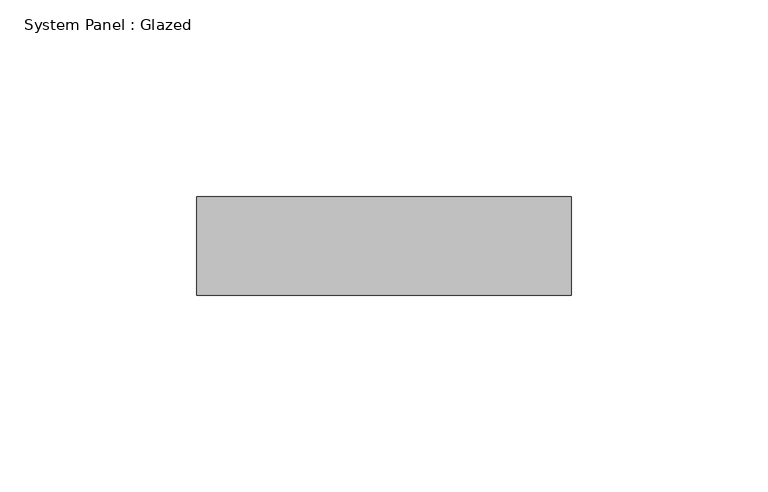
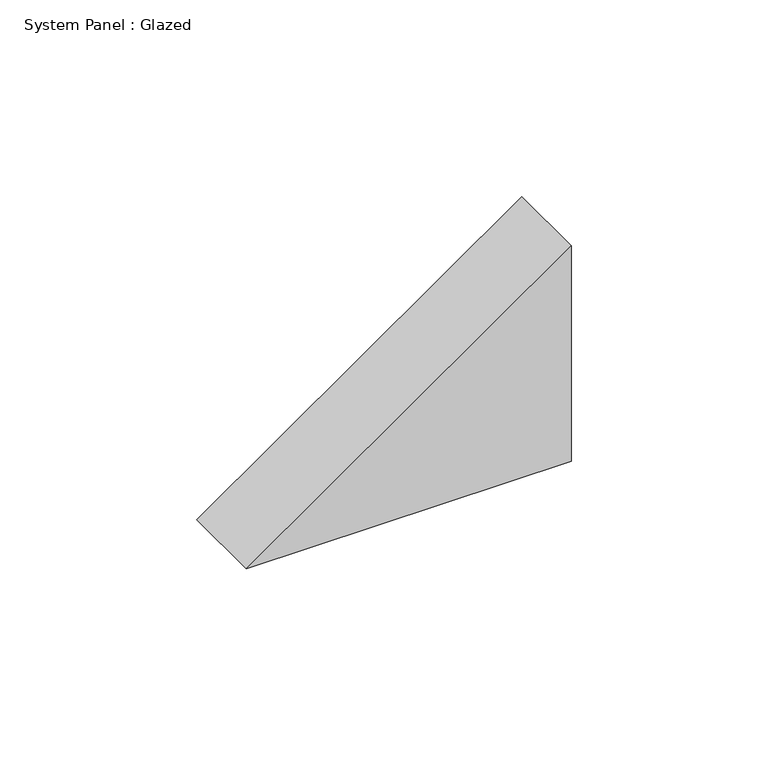
"""IFC4 building model written with IfcOpenShell, lengths in millimetres: plate geometry, System Panel : Glazed."""

from ifc_helpers import new_model, si_unit, frame, origin, place, context, project, spatial, polyline, outline, extrude, source, transform, mapped, element, save


def system_panel_glazed_45bde3df(model_context):
    return source(origin(), model_context, "Body", "SweptSolid", [
        extrude(outline(polyline([(0.0, -47.617578), (0.0, 47.617578), (66.6843741, 47.617578), (0.0, -47.617578)])), frame((0.0, 24.5, 0.0), z_axis=(0.0, 1.0, 0.0), x_axis=(0.0, 0.0, 1.0)), (0.0, 0.0, 1.0), 25.0),
    ])


if __name__ == "__main__":
    model = new_model("IFC4")
    model_context = context("Model", 3, world=origin())
    ifc_project = project(units=[si_unit("LENGTHUNIT", "METRE", prefix="MILLI")], contexts=[model_context])
    site = spatial("IfcSite", under=ifc_project)
    building = spatial("IfcBuilding", under=site)
    placement = place(None, origin())
    system_panel_glazed_shape = system_panel_glazed_45bde3df(model_context)
    element("IfcPlate", 1, ObjectType="System Panel : Glazed", at=placement, inside=building, context=model_context, shape_type="MappedRepresentation", body=[
        mapped(system_panel_glazed_shape, transform((0.0, 0.0, 0.0), x_axis=(1.0, 0.0, 0.0), y_axis=(0.0, 1.0, 0.0), z_axis=(0.0, 0.0, 1.0))),
    ])
    save(model, "model.ifc")

# Revit data of these elements
# Type "System Panel : Glazed"
#   Construction Type Id = "GSP4R"
#   Analytic Construction = "1/8 in Pilkington single glazing"
#   Visual Light Transmittance = 0.9
#   Solar Heat Gain Coefficient = 0.86
#   Heat Transfer Coefficient (U) = 6.7069 W/(m²·K)
#   Define Thermal Properties by = 1
# Element 1 (IfcPlate, "System Panel : Glazed")
#   Materials on its faces: "Glass"
# Materials
#   "Glass": class "Glass", colour RGB 0 128 192, transparency 0.9, Description = "Soda Lime Glass", Cost = 0
